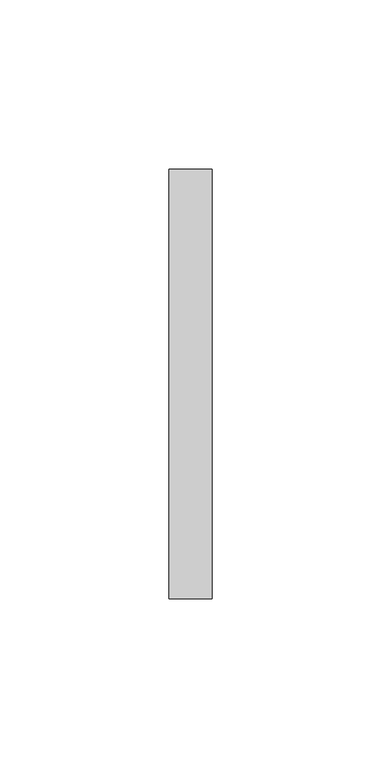
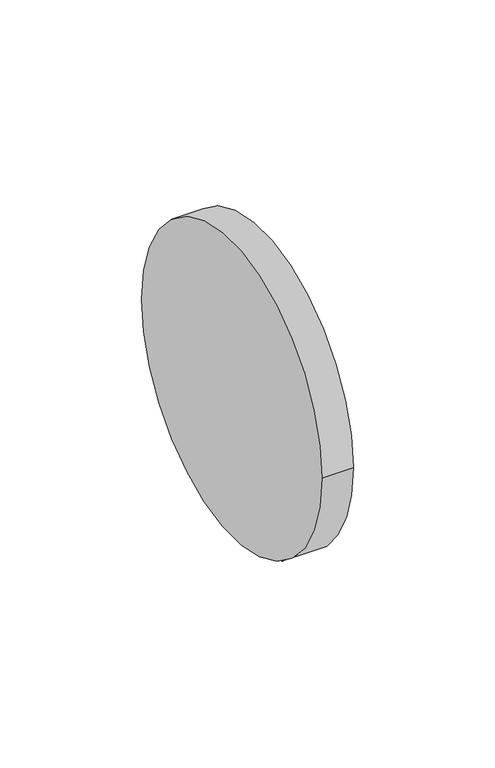
"""IFC4 building model written with IfcOpenShell, lengths in millimetres: proxy geometry, DOAS Supply to Return Connection : DOAS Supply to Return Duct Connection."""

from ifc_helpers import new_model, si_unit, point, frame, origin, origin_2d, place, context, project, spatial, circle_curve, trimmed, segment, composite_curve, outline, extrude, source, transform, mapped, element, save


def mechanical_equipment_142123ad(model_context):
    return source(origin(), model_context, "Body", "SweptSolid", [
        extrude(outline(composite_curve([segment(trimmed(circle_curve(origin_2d(), 63.5), [point((-63.5, 0.0))], [point((63.5, 0.0))], False, "CARTESIAN"), True, "CONTINUOUS"), segment(trimmed(circle_curve(origin_2d(), 63.5), [point((63.5, 0.0))], [point((-63.5, 0.0))], False, "CARTESIAN"), True, "CONTINUOUS")], self_intersect=False)), frame((0.0, 0.0, 0.0), z_axis=(1.0, 0.0, 0.0), x_axis=(0.0, 1.0, 0.0)), (0.0, 0.0, 1.0), 12.7),
    ])


if __name__ == "__main__":
    model = new_model("IFC4")
    model_context = context("Model", 3, world=origin())
    ifc_project = project(units=[si_unit("LENGTHUNIT", "METRE", prefix="MILLI")], contexts=[model_context])
    site = spatial("IfcSite", under=ifc_project)
    building = spatial("IfcBuilding", under=site)
    placement = place(None, origin())
    mechanical_equipment_shape = mechanical_equipment_142123ad(model_context)
    element("IfcBuildingElementProxy", 1, Name="DOAS Supply to Return Connection : DOAS Supply to Return Duct Connection", ObjectType="DOAS Supply to Return Connection : DOAS Supply to Return Duct Connection", at=placement, inside=building, context=model_context, shape_type="MappedRepresentation", body=[
        mapped(mechanical_equipment_shape, transform((0.0, 0.0, 0.0), x_axis=(1.0, 0.0, 0.0), y_axis=(0.0, 1.0, 0.0), z_axis=(0.0, 0.0, 1.0))),
    ])
    save(model, "model.ifc")

# Revit data of these elements
# Project information
#   Project Issue Date = "Issue Date"
#   Project Status = "Project Status"
#   Client Name = "Owner"
#   Project Address = "Enter address here"
#   Project Name = "Project Name"
#   Project Number = "Project Number"
# Type "DOAS Supply to Return Connection : DOAS Supply to Return Duct Connection"
#   Type Comments = "Generic Connector - no power"
#   Supply Side Airflow = 0 CFM
#   Return Side Airflow [instance default] = 0 CFM
#   Duct Connection [instance default] = 6"
#   Connector Length [instance default] = 0' - 0 1/2"
#   Default Elevation = 0
# Element 1 (IfcBuildingElementProxy, "DOAS Supply to Return Connection : DOAS Supply to Return Duct Connection")
#   Duct Connection = 5"
